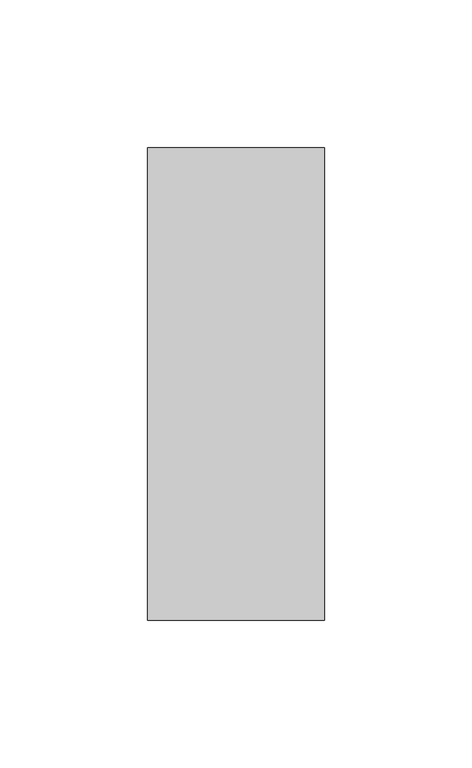
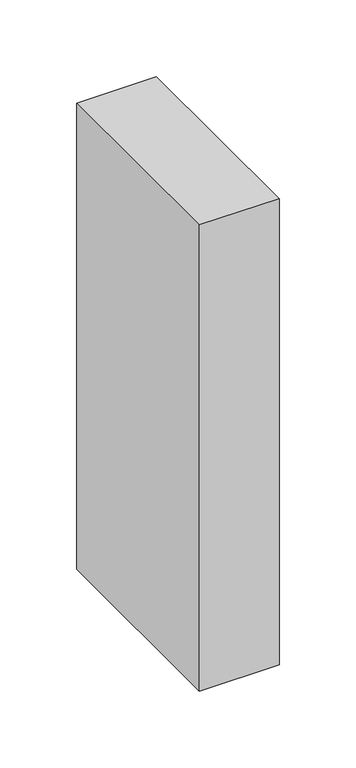
"""IFC4 building model written with IfcOpenShell, lengths in millimetres: column geometry, Madeira de lei-Coluna : Pontalete 6X16cm."""

from ifc_helpers import new_model, si_unit, frame, origin, place, context, project, spatial, polyline, outline, extrude, source, transform, mapped, element, save


def column_910cb117(model_context):
    return source(origin(), model_context, "Body", "SweptSolid", [
        extrude(outline(polyline([(30.0, 80.0), (30.0, -80.0), (-30.0, -80.0), (-30.0, 80.0), (30.0, 80.0)])), frame((0.0, 0.0, 6710.0), z_axis=(0.0, 0.0, 1.0), x_axis=(1.0, 0.0, 0.0)), (0.0, 0.0, 1.0), 371.3),
    ])


if __name__ == "__main__":
    model = new_model("IFC4")
    model_context = context("Model", 3, world=origin())
    ifc_project = project(units=[si_unit("LENGTHUNIT", "METRE", prefix="MILLI")], contexts=[model_context])
    site = spatial("IfcSite", under=ifc_project)
    building = spatial("IfcBuilding", under=site)
    placement = place(None, origin())
    column_shape = column_910cb117(model_context)
    element("IfcColumn", 1, ObjectType="Madeira de lei-Coluna : Pontalete 6X16cm", at=placement, inside=building, context=model_context, shape_type="MappedRepresentation", body=[
        mapped(column_shape, transform((0.0, 0.0, 0.0), x_axis=(1.0, 0.0, 0.0), y_axis=(0.0, 1.0, 0.0), z_axis=(0.0, 0.0, 1.0))),
    ])
    save(model, "model.ifc")

# Revit data of these elements
# Type "Madeira de lei-Coluna : Pontalete 6X16cm"
#   A = 0.01952 m²
#   b = 0.06 m
#   d = 0.16 m
#   Structural Material [instance default] = none
#   Assembly Code = ""
# Element 1 (IfcColumn, "Madeira de lei-Coluna : Pontalete 6X16cm")
#   Structural Material = .MADEIRAMENTO
#   Materials on its faces: ".MADEIRAMENTO"
# Materials
#   ".MADEIRAMENTO": class ".CC_MADEIRAS", colour RGB 212 179 113, transparency 0, Cost = 0
